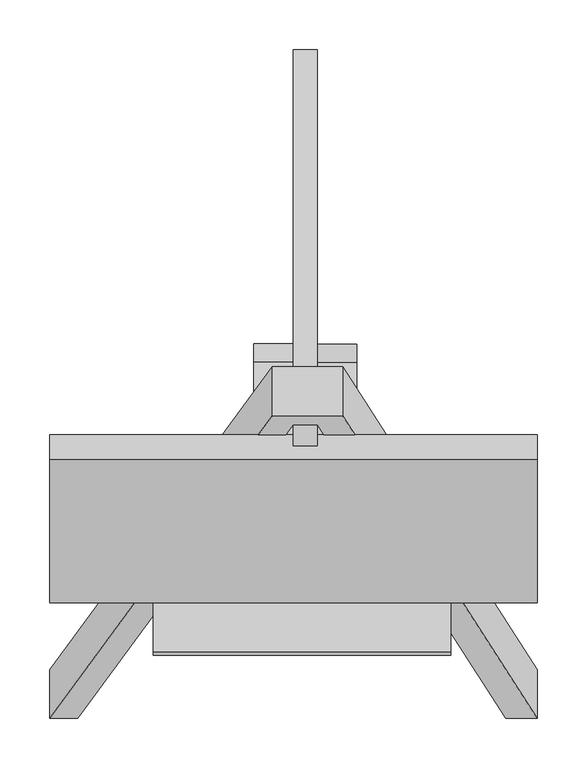
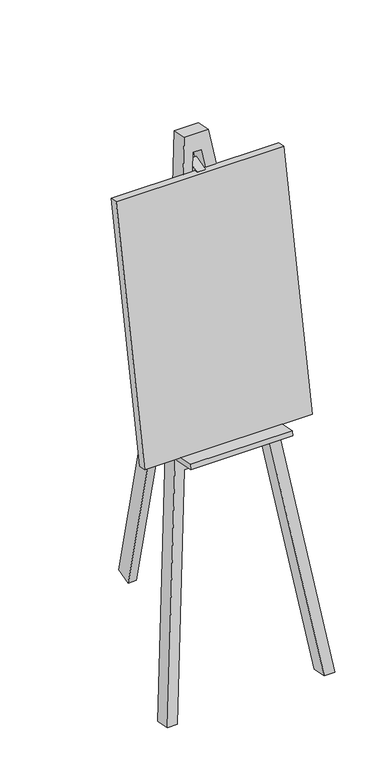
"""IFC4 building model written with IfcOpenShell, lengths in millimetres: furniture geometry, Caballete_Art_Easel_5160 : Caballete_Art_Easel_5160."""

from ifc_helpers import new_model, si_unit, point, frame, frame_2d, origin, place, context, project, spatial, polyline, circle_curve, trimmed, segment, composite_curve, outline, extrude, source, transform, mapped, element, save


def furniture_cf803cb7(model_context):
    return source(origin(), model_context, "Body", "SweptSolid", [
        extrude(outline(polyline([(0.0, -25.0), (0.0, 0.0), (492.1696373, 0.0), (492.1696373, -25.0), (0.0, -25.0)])), frame((163.6591839, 67.5766178, 740.7147904), z_axis=(0.0, 0.19080899537654755, 0.9816271834476635), x_axis=(-1.0, 0.0, 0.0)), (0.0, 0.0, 1.0), 758.2171145),
        extrude(outline(composite_curve([segment(polyline([(228.2886308, 1294.8913622), (310.3923261, 1272.8917434)]), True, "CONTINUOUS"), segment(trimmed(circle_curve(frame_2d((303.9218499, 1248.7435977)), 25.0), [point((310.3923261, 1272.8917434))], [point((297.4513738, 1224.5954521))], False, "CARTESIAN"), True, "CONTINUOUS"), segment(polyline([(297.4513738, 1224.5954521), (215.3476786, 1246.5950709)]), True, "CONTINUOUS"), segment(trimmed(circle_curve(frame_2d((221.8181547, 1270.7432166)), 25.0), [point((215.3476786, 1246.5950709))], [point((228.2886308, 1294.8913622))], False, "CARTESIAN"), True, "CONTINUOUS")], self_intersect=False)), frame((-122.5780911, 0.0, 0.0), z_axis=(1.0, 0.0, 0.0), x_axis=(0.0, 1.0, 0.0)), (0.0, 0.0, 1.0), 40.1524564),
        extrude(outline(composite_curve([segment(polyline([(227.8963048, 1294.8913622), (310.0, 1272.8917434)]), True, "CONTINUOUS"), segment(trimmed(circle_curve(frame_2d((303.5295239, 1248.7435977)), 25.0), [point((310.0, 1272.8917434))], [point((297.0590477, 1224.5954521))], False, "CARTESIAN"), True, "CONTINUOUS"), segment(polyline([(297.0590477, 1224.5954521), (214.9553525, 1246.5950709)]), True, "CONTINUOUS"), segment(trimmed(circle_curve(frame_2d((221.4258286, 1270.7432166)), 25.0), [point((214.9553525, 1246.5950709))], [point((227.8963048, 1294.8913622))], False, "CARTESIAN"), True, "CONTINUOUS")], self_intersect=False)), frame((-58.511631, 0.0, 0.0), z_axis=(1.0, 0.0, 0.0), x_axis=(0.0, 1.0, 0.0)), (0.0, 0.0, 1.0), 40.1524564),
        extrude(outline(polyline([(0.0, -76.0901602), (0.0, 0.0), (300.1179888, 0.0), (300.1179888, -76.0901602), (0.0, -76.0901602)])), frame((76.1864792, 14.6405989, 736.138093), z_axis=(0.0, 0.19080899537653903, 0.9816271834476651), x_axis=(-1.0, 0.0, 0.0)), (0.0, 0.0, 1.0), 14.5932792),
        extrude(outline(polyline([(0.0, -23.9729594), (0.0, 0.0), (50.0, 0.0), (50.0, -23.9729594), (0.0, -23.9729594)])), frame((-82.4845904, 576.9699849, -7.3165022), z_axis=(0.0, -0.23021547965360503, 0.9731396780153714), x_axis=(0.0, 0.9731396780153714, 0.23021547965360503)), (0.0, 0.0, 1.0), 1531.0625841),
        extrude(outline(polyline([(31.8547455, 0.0), (116.5760926, -690.0), (366.9499365, -690.0), (463.9231124, 0.0), (492.1696373, 0.0), (267.3043017, -1600.0), (196.4552974, -1600.0), (0.0, 0.0), (31.8547455, 0.0)]), holes=[polyline([(222.1708149, -1550.0), (246.0848186, -1550.0), (359.9228947, -740.0000001), (122.7153206, -740.0000001), (222.1708149, -1550.0)])]), frame((163.6591839, 0.0, 0.0), z_axis=(0.0, -0.9816271834476651, 0.190808995376539), x_axis=(-1.0, 0.0, 0.0)), (0.0, 0.0, 1.0), 50.0),
    ])


if __name__ == "__main__":
    model = new_model("IFC4")
    model_context = context("Model", 3, world=origin())
    ifc_project = project(units=[si_unit("LENGTHUNIT", "METRE", prefix="MILLI")], contexts=[model_context])
    site = spatial("IfcSite", under=ifc_project)
    building = spatial("IfcBuilding", under=site)
    placement = place(None, origin())
    furniture_shape = furniture_cf803cb7(model_context)
    element("IfcFurniture", 1, ObjectType="Caballete_Art_Easel_5160 : Caballete_Art_Easel_5160", at=placement, inside=building, context=model_context, shape_type="MappedRepresentation", body=[
        mapped(furniture_shape, transform((0.0, 0.0, 0.0), x_axis=(1.0, 0.0, 0.0), y_axis=(0.0, 1.0, 0.0), z_axis=(0.0, 0.0, 1.0))),
    ])
    save(model, "model.ifc")

# Revit data of these elements
# Type "Caballete_Art_Easel_5160 : Caballete_Art_Easel_5160"
#   Default Elevation = 0
# Element 1 (IfcFurniture, "Caballete_Art_Easel_5160 : Caballete_Art_Easel_5160")
#   Materials on its faces: "Madera", "Lienzo"
# Materials
#   "Madera": class "Unassigned", colour RGB 212 179 113, transparency 0
#   "Lienzo": class "Unassigned", colour RGB 251 251 251, transparency 0
